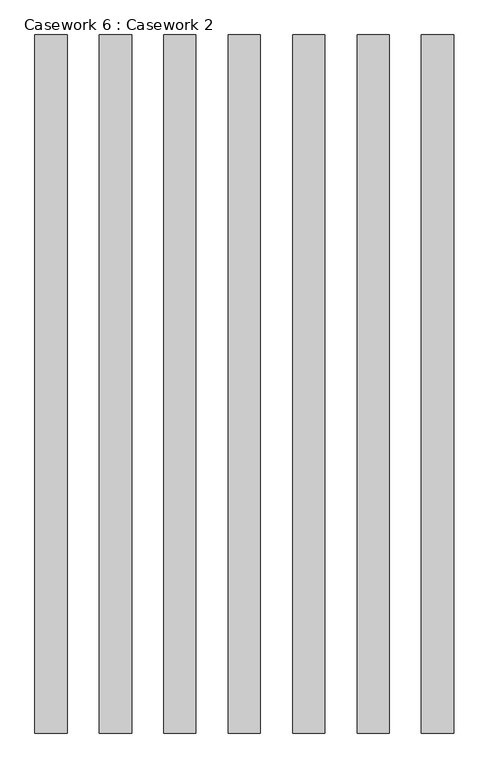
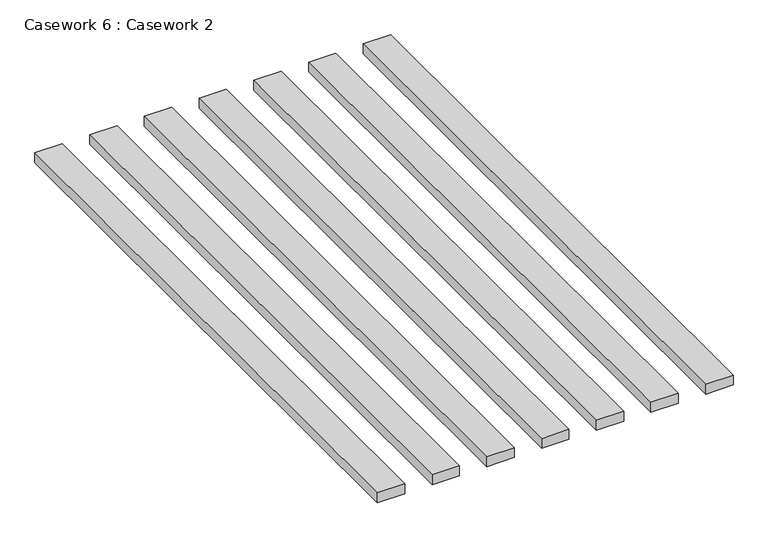
"""IFC4 building model written with IfcOpenShell, lengths in millimetres: furniture geometry, Casework 6 : Casework 2."""

import ifcopenshell
import ifcopenshell.guid

model = None  # the IFC model being written
_history = None  # IfcOwnerHistory: only IFC2X3 demands one
_inside = {}  # id of a spatial element -> (the spatial element, [elements in it])
_under = {}  # id of a project, library or spatial element -> (it, [spatial elements below it])
_declared = {}  # id of a project -> (the project, [libraries it declares])
_typed = {}  # id of a type object -> (the type object, [elements of that type])
_made_of = {}  # id of a material, layer set ... -> (it, [elements and type objects made of it])


def new_model(schema):
    """Start an empty IFC model of exactly this schema.

    Asked for "IFC4X3", IfcOpenShell would pick the latest addendum, in which some entities
    have other attributes; the version numbers below select the first issue.
    IFC2X3 requires an IfcOwnerHistory on every rooted entity: one is made here for all.
    """
    global model, _history
    if schema == "IFC4X3":
        model = ifcopenshell.file(schema_version=(4, 3, 0, 0))
    else:
        model = ifcopenshell.file(schema=schema)
    _inside.clear()
    _under.clear()
    _declared.clear()
    _typed.clear()
    _made_of.clear()
    _history = None
    if model.schema == "IFC2X3":
        org = make("IfcOrganization", Name="unknown")
        user = make(
            "IfcPersonAndOrganization",
            ThePerson=make("IfcPerson", FamilyName="unknown"),
            TheOrganization=org,
        )
        app = make(
            "IfcApplication",
            ApplicationDeveloper=org,
            Version="unknown",
            ApplicationFullName="unknown",
            ApplicationIdentifier="unknown",
        )
        _history = make(
            "IfcOwnerHistory",
            OwningUser=user,
            OwningApplication=app,
            ChangeAction="ADDED",
            CreationDate=0,
        )
    return model


def make(cls, **values):
    """One entity of the class cls with the attributes given. An attribute that is None is left unset."""
    return model.create_entity(
        cls, **{name: value for name, value in values.items() if value is not None}
    )


def rooted(cls, **values):
    """An entity with a GlobalId (a new one), such as an element, a storey or a relation."""
    return make(cls, GlobalId=ifcopenshell.guid.new(), OwnerHistory=_history, **values)


def si_unit(unit_type, name, prefix=None):
    """IfcSIUnit, for example si_unit("LENGTHUNIT", "METRE", prefix="MILLI")."""
    return make("IfcSIUnit", UnitType=unit_type, Prefix=prefix, Name=name)


def assignment(units):
    """IfcUnitAssignment: the units of a project."""
    return None if units is None else make("IfcUnitAssignment", Units=units)


def point(xyz):
    """IfcCartesianPoint."""
    return None if xyz is None else make("IfcCartesianPoint", Coordinates=xyz)


def direction(xyz):
    """IfcDirection."""
    return None if xyz is None else make("IfcDirection", DirectionRatios=xyz)


def frame(location, z_axis=None, x_axis=None):
    """IfcAxis2Placement3D, a coordinate frame: its origin and axes. An axis left out is left unset."""
    return make(
        "IfcAxis2Placement3D",
        Location=point(location),
        Axis=direction(z_axis),
        RefDirection=direction(x_axis),
    )


def origin():
    """The frame at (0, 0, 0) with its axes left unset."""
    return frame((0.0, 0.0, 0.0))


def place(relative_to, where):
    """IfcLocalPlacement: puts the frame where relative to a parent placement (None: the world)."""
    return make(
        "IfcLocalPlacement", PlacementRelTo=relative_to, RelativePlacement=where
    )


def context(
    kind, dimensions, precision=None, world=None, true_north=None, identifier=None
):
    """IfcGeometricRepresentationContext, for example the 3D "Model" context."""
    return make(
        "IfcGeometricRepresentationContext",
        ContextIdentifier=identifier,
        ContextType=kind,
        CoordinateSpaceDimension=dimensions,
        Precision=precision,
        WorldCoordinateSystem=world,
        TrueNorth=true_north,
    )


def project(units=None, contexts=None):
    """IfcProject with its units and contexts."""
    return rooted(
        "IfcProject",
        Name="project",
        RepresentationContexts=contexts,
        UnitsInContext=assignment(units),
    )


def spatial(cls, under=None, at=None, **own):
    """A site, building, storey or space (cls), placed at a placement, below another one or the project."""
    s = rooted(cls, ObjectPlacement=at, **own)
    if under is not None:
        _under.setdefault(under.id(), (under, []))[1].append(s)
    return s


def polyline(points):
    """IfcPolyline through the points."""
    return make("IfcPolyline", Points=[point(p) for p in points])


def outline(outer, holes=None, kind="AREA"):
    """IfcArbitraryClosedProfileDef: a profile drawn as a closed curve; with holes, ...WithVoids."""
    if holes is None:
        return make("IfcArbitraryClosedProfileDef", ProfileType=kind, OuterCurve=outer)
    return make(
        "IfcArbitraryProfileDefWithVoids",
        ProfileType=kind,
        OuterCurve=outer,
        InnerCurves=holes,
    )


def extrude(swept, where, along, depth):
    """IfcExtrudedAreaSolid: the profile swept, set in the frame where, extruded along a direction by depth."""
    return make(
        "IfcExtrudedAreaSolid",
        SweptArea=swept,
        Position=where,
        ExtrudedDirection=direction(along),
        Depth=depth,
    )


def shape(context_of_items, identifier, shape_type, items):
    """IfcShapeRepresentation: the items that make up one representation, for example the "Body"."""
    return make(
        "IfcShapeRepresentation",
        ContextOfItems=context_of_items,
        RepresentationIdentifier=identifier,
        RepresentationType=shape_type,
        Items=items,
    )


def source(mapping_origin, context_of_items, identifier, shape_type, items):
    """IfcRepresentationMap: a shape defined once, which mapped items show again and again."""
    return make(
        "IfcRepresentationMap",
        MappingOrigin=mapping_origin,
        MappedRepresentation=shape(context_of_items, identifier, shape_type, items),
    )


def transform(
    local_origin,
    x_axis=None,
    y_axis=None,
    z_axis=None,
    scale=None,
    scale2=None,
    scale3=None,
    uniform=True,
):
    """IfcCartesianTransformationOperator3D, or its non-uniform kind. x_axis, y_axis, z_axis: its Axis1, 2, 3."""
    if uniform:
        return make(
            "IfcCartesianTransformationOperator3D",
            Axis1=direction(x_axis),
            Axis2=direction(y_axis),
            LocalOrigin=point(local_origin),
            Scale=scale,
            Axis3=direction(z_axis),
        )
    return make(
        "IfcCartesianTransformationOperator3DnonUniform",
        Axis1=direction(x_axis),
        Axis2=direction(y_axis),
        LocalOrigin=point(local_origin),
        Scale=scale,
        Axis3=direction(z_axis),
        Scale2=scale2,
        Scale3=scale3,
    )


def mapped(mapping_source, mapping_target):
    """IfcMappedItem: shows the shape of a source again, moved by a transform."""
    return make(
        "IfcMappedItem", MappingSource=mapping_source, MappingTarget=mapping_target
    )


def made_of(thing, what):
    """Note that an element or type object is made of a material, layer set ...; save() writes the relation."""
    if what is not None:
        _made_of.setdefault(what.id(), (what, []))[1].append(thing)
    return thing


def element(
    cls,
    number,
    at=None,
    inside=None,
    cuts=None,
    type_object=None,
    material=None,
    context=None,
    identifier="Body",
    shape_type=None,
    held_by="IfcProductDefinitionShape",
    body=None,
    shapes=None,
    **own,
):
    """One element of the class cls, such as IfcWall. Its Tag is "e" and its number.

    at: its placement. inside: the storey or other place that contains it. cuts: it is an
    opening in that element (IfcRelVoidsElement). A single representation is given by context,
    identifier, shape_type and body (its items); several are given by shapes. held_by: the class
    of the entity that holds the representations. save() writes the other relations.
    """
    e = rooted(cls, Tag="e%d" % number, ObjectPlacement=at, **own)
    if body is not None:
        shapes = [shape(context, identifier, shape_type, body)]
    if shapes is not None:
        e.Representation = make(held_by, Representations=shapes)
    if inside is not None:
        _inside.setdefault(inside.id(), (inside, []))[1].append(e)
    if cuts is not None:
        rooted(
            "IfcRelVoidsElement", RelatingBuildingElement=cuts, RelatedOpeningElement=e
        )
    if type_object is not None:
        _typed.setdefault(type_object.id(), (type_object, []))[1].append(e)
    return made_of(e, material)


def aggregate(whole, parts):
    """IfcRelAggregates: a whole, such as a stair, and the parts it consists of."""
    return rooted("IfcRelAggregates", RelatingObject=whole, RelatedObjects=parts)


def save(model, path):
    """Write the relations noted so far, then the file.

    IfcRelAggregates (storeys below a building ...), IfcRelContainedInSpatialStructure (elements
    in a storey), IfcRelDefinesByType, IfcRelAssociatesMaterial and IfcRelDeclares: one each for
    every whole, place, type object, material and project.
    """
    for whole, parts in _under.values():
        aggregate(whole, parts)
    for where, things in _inside.values():
        rooted(
            "IfcRelContainedInSpatialStructure",
            RelatedElements=things,
            RelatingStructure=where,
        )
    for kind, things in _typed.values():
        rooted("IfcRelDefinesByType", RelatedObjects=things, RelatingType=kind)
    for what, things in _made_of.values():
        rooted("IfcRelAssociatesMaterial", RelatedObjects=things, RelatingMaterial=what)
    for by, libraries in _declared.values():
        rooted("IfcRelDeclares", RelatingContext=by, RelatedDefinitions=libraries)
    model.write(path)


def casework_6_casework_2_13822944(model_context):
    return source(origin(), model_context, "Body", "SweptSolid", [
        extrude(outline(polyline([(-4948.5247381, 2870.3649316), (-4898.5247381, 2870.3649316), (-4898.5247381, 1786.6149316), (-4948.5247381, 1786.6149316), (-4948.5247381, 2870.3649316)])), frame((0.0, 0.0, 4033.1977901), z_axis=(0.0, 0.0, 1.0), x_axis=(1.0, 0.0, 0.0)), (0.0, 0.0, 1.0), 19.0),
        extrude(outline(polyline([(-4848.5247381, 2870.3649316), (-4798.5247381, 2870.3649316), (-4798.5247381, 1786.6149316), (-4848.5247381, 1786.6149316), (-4848.5247381, 2870.3649316)])), frame((0.0, 0.0, 4033.1977901), z_axis=(0.0, 0.0, 1.0), x_axis=(1.0, 0.0, 0.0)), (0.0, 0.0, 1.0), 19.0),
        extrude(outline(polyline([(-4748.5247381, 2870.3649316), (-4698.5247381, 2870.3649316), (-4698.5247381, 1786.6149316), (-4748.5247381, 1786.6149316), (-4748.5247381, 2870.3649316)])), frame((0.0, 0.0, 4033.1977901), z_axis=(0.0, 0.0, 1.0), x_axis=(1.0, 0.0, 0.0)), (0.0, 0.0, 1.0), 19.0),
        extrude(outline(polyline([(-4648.5247381, 2870.3649316), (-4598.5247381, 2870.3649316), (-4598.5247381, 1786.6149316), (-4648.5247381, 1786.6149316), (-4648.5247381, 2870.3649316)])), frame((0.0, 0.0, 4033.1977901), z_axis=(0.0, 0.0, 1.0), x_axis=(1.0, 0.0, 0.0)), (0.0, 0.0, 1.0), 19.0),
        extrude(outline(polyline([(-4548.5247381, 2870.3649316), (-4498.5247381, 2870.3649316), (-4498.5247381, 1786.6149316), (-4548.5247381, 1786.6149316), (-4548.5247381, 2870.3649316)])), frame((0.0, 0.0, 4033.1977901), z_axis=(0.0, 0.0, 1.0), x_axis=(1.0, 0.0, 0.0)), (0.0, 0.0, 1.0), 19.0),
        extrude(outline(polyline([(-4448.5247381, 2870.3649316), (-4398.5247381, 2870.3649316), (-4398.5247381, 1786.6149316), (-4448.5247381, 1786.6149316), (-4448.5247381, 2870.3649316)])), frame((0.0, 0.0, 4033.1977901), z_axis=(0.0, 0.0, 1.0), x_axis=(1.0, 0.0, 0.0)), (0.0, 0.0, 1.0), 19.0),
        extrude(outline(polyline([(-4348.5247381, 2870.3649316), (-4298.5247381, 2870.3649316), (-4298.5247381, 1786.6149316), (-4348.5247381, 1786.6149316), (-4348.5247381, 2870.3649316)])), frame((0.0, 0.0, 4033.1977901), z_axis=(0.0, 0.0, 1.0), x_axis=(1.0, 0.0, 0.0)), (0.0, 0.0, 1.0), 19.0),
    ])


if __name__ == "__main__":
    model = new_model("IFC4")
    model_context = context("Model", 3, world=origin())
    ifc_project = project(units=[si_unit("LENGTHUNIT", "METRE", prefix="MILLI")], contexts=[model_context])
    site = spatial("IfcSite", under=ifc_project)
    building = spatial("IfcBuilding", under=site)
    placement = place(None, origin())
    casework_6_casework_2_shape = casework_6_casework_2_13822944(model_context)
    element("IfcFurniture", 1, ObjectType="Casework 6 : Casework 2", at=placement, inside=building, context=model_context, shape_type="MappedRepresentation", body=[
        mapped(casework_6_casework_2_shape, transform((0.0, 0.0, 0.0), x_axis=(1.0, 0.0, 0.0), y_axis=(0.0, 1.0, 0.0), z_axis=(0.0, 0.0, 1.0))),
    ])
    save(model, "model.ifc")
